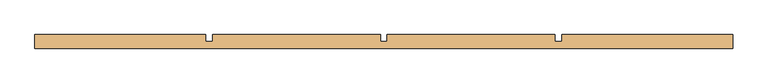
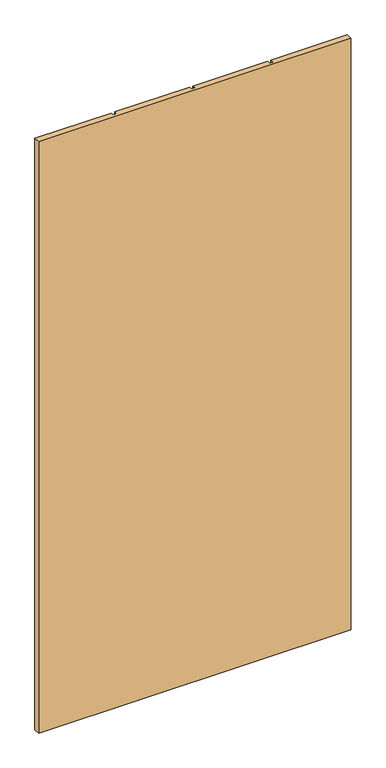
"""IFC4 building model written with IfcOpenShell, lengths in millimetres: door geometry, BA_Bi-fold door : AD_Bi-fold door - 100cm."""

import ifcopenshell
import ifcopenshell.guid

model = None  # the IFC model being written
_history = None  # IfcOwnerHistory: only IFC2X3 demands one
_inside = {}  # id of a spatial element -> (the spatial element, [elements in it])
_under = {}  # id of a project, library or spatial element -> (it, [spatial elements below it])
_declared = {}  # id of a project -> (the project, [libraries it declares])
_typed = {}  # id of a type object -> (the type object, [elements of that type])
_made_of = {}  # id of a material, layer set ... -> (it, [elements and type objects made of it])


def new_model(schema):
    """Start an empty IFC model of exactly this schema.

    Asked for "IFC4X3", IfcOpenShell would pick the latest addendum, in which some entities
    have other attributes; the version numbers below select the first issue.
    IFC2X3 requires an IfcOwnerHistory on every rooted entity: one is made here for all.
    """
    global model, _history
    if schema == "IFC4X3":
        model = ifcopenshell.file(schema_version=(4, 3, 0, 0))
    else:
        model = ifcopenshell.file(schema=schema)
    _inside.clear()
    _under.clear()
    _declared.clear()
    _typed.clear()
    _made_of.clear()
    _history = None
    if model.schema == "IFC2X3":
        org = make("IfcOrganization", Name="unknown")
        user = make(
            "IfcPersonAndOrganization",
            ThePerson=make("IfcPerson", FamilyName="unknown"),
            TheOrganization=org,
        )
        app = make(
            "IfcApplication",
            ApplicationDeveloper=org,
            Version="unknown",
            ApplicationFullName="unknown",
            ApplicationIdentifier="unknown",
        )
        _history = make(
            "IfcOwnerHistory",
            OwningUser=user,
            OwningApplication=app,
            ChangeAction="ADDED",
            CreationDate=0,
        )
    return model


def make(cls, **values):
    """One entity of the class cls with the attributes given. An attribute that is None is left unset."""
    return model.create_entity(
        cls, **{name: value for name, value in values.items() if value is not None}
    )


def rooted(cls, **values):
    """An entity with a GlobalId (a new one), such as an element, a storey or a relation."""
    return make(cls, GlobalId=ifcopenshell.guid.new(), OwnerHistory=_history, **values)


def si_unit(unit_type, name, prefix=None):
    """IfcSIUnit, for example si_unit("LENGTHUNIT", "METRE", prefix="MILLI")."""
    return make("IfcSIUnit", UnitType=unit_type, Prefix=prefix, Name=name)


def assignment(units):
    """IfcUnitAssignment: the units of a project."""
    return None if units is None else make("IfcUnitAssignment", Units=units)


def point(xyz):
    """IfcCartesianPoint."""
    return None if xyz is None else make("IfcCartesianPoint", Coordinates=xyz)


def direction(xyz):
    """IfcDirection."""
    return None if xyz is None else make("IfcDirection", DirectionRatios=xyz)


def frame(location, z_axis=None, x_axis=None):
    """IfcAxis2Placement3D, a coordinate frame: its origin and axes. An axis left out is left unset."""
    return make(
        "IfcAxis2Placement3D",
        Location=point(location),
        Axis=direction(z_axis),
        RefDirection=direction(x_axis),
    )


def origin():
    """The frame at (0, 0, 0) with its axes left unset."""
    return frame((0.0, 0.0, 0.0))


def origin_with_axes():
    """The frame at (0, 0, 0) with the z axis (0, 0, 1) and the x axis (1, 0, 0) written out."""
    return frame((0.0, 0.0, 0.0), z_axis=(0.0, 0.0, 1.0), x_axis=(1.0, 0.0, 0.0))


def place(relative_to, where):
    """IfcLocalPlacement: puts the frame where relative to a parent placement (None: the world)."""
    return make(
        "IfcLocalPlacement", PlacementRelTo=relative_to, RelativePlacement=where
    )


def context(
    kind, dimensions, precision=None, world=None, true_north=None, identifier=None
):
    """IfcGeometricRepresentationContext, for example the 3D "Model" context."""
    return make(
        "IfcGeometricRepresentationContext",
        ContextIdentifier=identifier,
        ContextType=kind,
        CoordinateSpaceDimension=dimensions,
        Precision=precision,
        WorldCoordinateSystem=world,
        TrueNorth=true_north,
    )


def project(units=None, contexts=None):
    """IfcProject with its units and contexts."""
    return rooted(
        "IfcProject",
        Name="project",
        RepresentationContexts=contexts,
        UnitsInContext=assignment(units),
    )


def spatial(cls, under=None, at=None, **own):
    """A site, building, storey or space (cls), placed at a placement, below another one or the project."""
    s = rooted(cls, ObjectPlacement=at, **own)
    if under is not None:
        _under.setdefault(under.id(), (under, []))[1].append(s)
    return s


def polyline(points):
    """IfcPolyline through the points."""
    return make("IfcPolyline", Points=[point(p) for p in points])


def outline(outer, holes=None, kind="AREA"):
    """IfcArbitraryClosedProfileDef: a profile drawn as a closed curve; with holes, ...WithVoids."""
    if holes is None:
        return make("IfcArbitraryClosedProfileDef", ProfileType=kind, OuterCurve=outer)
    return make(
        "IfcArbitraryProfileDefWithVoids",
        ProfileType=kind,
        OuterCurve=outer,
        InnerCurves=holes,
    )


def extrude(swept, where, along, depth):
    """IfcExtrudedAreaSolid: the profile swept, set in the frame where, extruded along a direction by depth."""
    return make(
        "IfcExtrudedAreaSolid",
        SweptArea=swept,
        Position=where,
        ExtrudedDirection=direction(along),
        Depth=depth,
    )


def shape(context_of_items, identifier, shape_type, items):
    """IfcShapeRepresentation: the items that make up one representation, for example the "Body"."""
    return make(
        "IfcShapeRepresentation",
        ContextOfItems=context_of_items,
        RepresentationIdentifier=identifier,
        RepresentationType=shape_type,
        Items=items,
    )


def source(mapping_origin, context_of_items, identifier, shape_type, items):
    """IfcRepresentationMap: a shape defined once, which mapped items show again and again."""
    return make(
        "IfcRepresentationMap",
        MappingOrigin=mapping_origin,
        MappedRepresentation=shape(context_of_items, identifier, shape_type, items),
    )


def transform(
    local_origin,
    x_axis=None,
    y_axis=None,
    z_axis=None,
    scale=None,
    scale2=None,
    scale3=None,
    uniform=True,
):
    """IfcCartesianTransformationOperator3D, or its non-uniform kind. x_axis, y_axis, z_axis: its Axis1, 2, 3."""
    if uniform:
        return make(
            "IfcCartesianTransformationOperator3D",
            Axis1=direction(x_axis),
            Axis2=direction(y_axis),
            LocalOrigin=point(local_origin),
            Scale=scale,
            Axis3=direction(z_axis),
        )
    return make(
        "IfcCartesianTransformationOperator3DnonUniform",
        Axis1=direction(x_axis),
        Axis2=direction(y_axis),
        LocalOrigin=point(local_origin),
        Scale=scale,
        Axis3=direction(z_axis),
        Scale2=scale2,
        Scale3=scale3,
    )


def mapped(mapping_source, mapping_target):
    """IfcMappedItem: shows the shape of a source again, moved by a transform."""
    return make(
        "IfcMappedItem", MappingSource=mapping_source, MappingTarget=mapping_target
    )


def made_of(thing, what):
    """Note that an element or type object is made of a material, layer set ...; save() writes the relation."""
    if what is not None:
        _made_of.setdefault(what.id(), (what, []))[1].append(thing)
    return thing


def element(
    cls,
    number,
    at=None,
    inside=None,
    cuts=None,
    type_object=None,
    material=None,
    context=None,
    identifier="Body",
    shape_type=None,
    held_by="IfcProductDefinitionShape",
    body=None,
    shapes=None,
    **own,
):
    """One element of the class cls, such as IfcWall. Its Tag is "e" and its number.

    at: its placement. inside: the storey or other place that contains it. cuts: it is an
    opening in that element (IfcRelVoidsElement). A single representation is given by context,
    identifier, shape_type and body (its items); several are given by shapes. held_by: the class
    of the entity that holds the representations. save() writes the other relations.
    """
    e = rooted(cls, Tag="e%d" % number, ObjectPlacement=at, **own)
    if body is not None:
        shapes = [shape(context, identifier, shape_type, body)]
    if shapes is not None:
        e.Representation = make(held_by, Representations=shapes)
    if inside is not None:
        _inside.setdefault(inside.id(), (inside, []))[1].append(e)
    if cuts is not None:
        rooted(
            "IfcRelVoidsElement", RelatingBuildingElement=cuts, RelatedOpeningElement=e
        )
    if type_object is not None:
        _typed.setdefault(type_object.id(), (type_object, []))[1].append(e)
    return made_of(e, material)


def aggregate(whole, parts):
    """IfcRelAggregates: a whole, such as a stair, and the parts it consists of."""
    return rooted("IfcRelAggregates", RelatingObject=whole, RelatedObjects=parts)


def save(model, path):
    """Write the relations noted so far, then the file.

    IfcRelAggregates (storeys below a building ...), IfcRelContainedInSpatialStructure (elements
    in a storey), IfcRelDefinesByType, IfcRelAssociatesMaterial and IfcRelDeclares: one each for
    every whole, place, type object, material and project.
    """
    for whole, parts in _under.values():
        aggregate(whole, parts)
    for where, things in _inside.values():
        rooted(
            "IfcRelContainedInSpatialStructure",
            RelatedElements=things,
            RelatingStructure=where,
        )
    for kind, things in _typed.values():
        rooted("IfcRelDefinesByType", RelatedObjects=things, RelatingType=kind)
    for what, things in _made_of.values():
        rooted("IfcRelAssociatesMaterial", RelatedObjects=things, RelatingMaterial=what)
    for by, libraries in _declared.values():
        rooted("IfcRelDeclares", RelatingContext=by, RelatedDefinitions=libraries)
    model.write(path)


def door_88445510(model_context):
    return source(origin(), model_context, "Body", "SweptSolid", [
        extrude(outline(polyline([(255.0, 10.0), (500.0, 10.0), (500.0, -10.0), (-500.0, -10.0), (-500.0, 10.0), (-255.0, 10.0), (-255.0, 0.0), (-245.0, 0.0), (-245.0, 10.0), (-5.0, 10.0), (-5.0, 0.0), (5.0, 0.0), (5.0, 10.0), (245.0, 10.0), (245.0, 0.0), (255.0, 0.0), (255.0, 10.0)])), origin_with_axes(), (0.0, 0.0, 1.0), 2000.0),
    ])


if __name__ == "__main__":
    model = new_model("IFC4")
    model_context = context("Model", 3, world=origin())
    ifc_project = project(units=[si_unit("LENGTHUNIT", "METRE", prefix="MILLI")], contexts=[model_context])
    site = spatial("IfcSite", under=ifc_project)
    building = spatial("IfcBuilding", under=site)
    placement = place(None, origin())
    door_shape = door_88445510(model_context)
    element("IfcDoor", 1, ObjectType="BA_Bi-fold door : AD_Bi-fold door - 100cm", at=placement, inside=building, context=model_context, shape_type="MappedRepresentation", body=[
        mapped(door_shape, transform((0.0, 0.0, 0.0), x_axis=(1.0, 0.0, 0.0), y_axis=(0.0, 1.0, 0.0), z_axis=(0.0, 0.0, 1.0))),
    ])
    save(model, "model.ifc")

# Revit data of these elements
# Type "BA_Bi-fold door : AD_Bi-fold door - 100cm"
#   Type Mark = "45"
#   Frame Projection Ext. = 25 mm
#   Frame Projection Int. = 25 mm
#   Frame Width = 75 mm
#   Height = 2000 mm
#   Width = 1000 mm
#   Define Thermal Properties by = 1
#   160cm = no
#   140cm = no
#   120cm = no
#   100cm = yes
#   Function = (empty or 0)
#   Wall Closure = (empty or 0)
# Element 1 (IfcDoor, "BA_Bi-fold door : AD_Bi-fold door - 100cm")
#   Materials on its faces: "Default"
# Materials
#   "Default": class "Generic", colour RGB 255 255 255, transparency 0, Cost = 0
